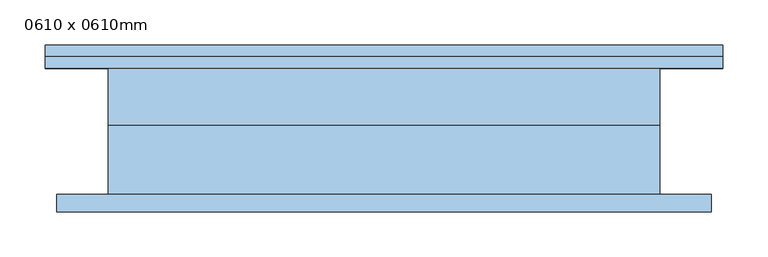
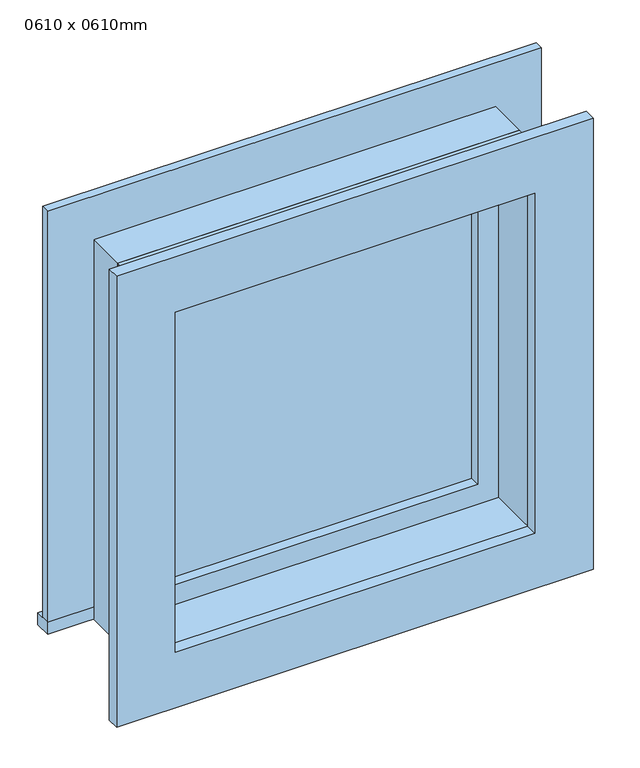
"""IFC4 building model written with IfcOpenShell, lengths in millimetres: window geometry, Travessa horizontal : 0610 x 0610mm."""

from ifc_helpers import new_model, si_unit, frame, origin, place, context, project, spatial, polyline, outline, extrude, source, transform, mapped, element, save


def window_0610_x_0610mm_59f802eb(model_context):
    return source(origin(), model_context, "Body", "SweptSolid", [
        extrude(outline(polyline([(-413.05, 95.7), (336.85, 95.7), (336.85, 70.0), (-413.05, 70.0), (-413.05, 95.7)])), frame((0.0, 0.0, 2159.0), z_axis=(0.0, 0.0, 1.0), x_axis=(1.0, 0.0, 0.0)), (0.0, 0.0, 1.0), 19.05),
        extrude(outline(polyline([(2749.95, -324.05), (2749.95, 247.85), (2178.05, 247.85), (2178.05, 336.85), (2838.95, 336.85), (2838.95, -413.05), (2178.05, -413.05), (2178.05, -324.05), (2749.95, -324.05)])), frame((0.0, 70.0, 0.0), z_axis=(0.0, 1.0, 0.0), x_axis=(0.0, 0.0, 1.0)), (0.0, 0.0, 1.0), 13.0),
        extrude(outline(polyline([(2826.25, 324.15), (2826.25, -400.35), (2101.75, -400.35), (2101.75, 324.15), (2826.25, 324.15)]), holes=[polyline([(2737.25, 235.15), (2190.75, 235.15), (2190.75, -311.35), (2737.25, -311.35), (2737.25, 235.15)])]), frame((0.0, -89.0, 0.0), z_axis=(0.0, 1.0, 0.0), x_axis=(0.0, 0.0, 1.0)), (0.0, 0.0, 1.0), 19.0),
        extrude(outline(polyline([(203.4, 22.425), (-279.6, 22.425), (-279.6, 35.125), (203.4, 35.125), (203.4, 22.425)])), frame((0.0, 0.0, 2222.5), z_axis=(0.0, 0.0, 1.0), x_axis=(1.0, 0.0, 0.0)), (0.0, 0.0, 1.0), 483.0),
        extrude(outline(polyline([(2749.95, -324.05), (2178.05, -324.05), (2178.05, 247.85), (2749.95, 247.85), (2749.95, -324.05)]), holes=[polyline([(2705.5, -279.6), (2705.5, 203.4), (2222.5, 203.4), (2222.5, -279.6), (2705.5, -279.6)])]), frame((0.0, 6.55, 0.0), z_axis=(0.0, 1.0, 0.0), x_axis=(0.0, 0.0, 1.0)), (0.0, 0.0, 1.0), 44.45),
        extrude(outline(polyline([(2769.0, -343.1), (2159.0, -343.1), (2159.0, 266.9), (2769.0, 266.9), (2769.0, -343.1)]), holes=[polyline([(2737.25, -311.35), (2737.25, 235.15), (2190.75, 235.15), (2190.75, -311.35), (2737.25, -311.35)])]), frame((0.0, -70.0, 0.0), z_axis=(0.0, 1.0, 0.0), x_axis=(0.0, 0.0, 1.0)), (0.0, 0.0, 1.0), 76.55),
        extrude(outline(polyline([(2769.0, 266.9), (2769.0, -343.1), (2159.0, -343.1), (2159.0, 266.9), (2769.0, 266.9)]), holes=[polyline([(2749.95, 247.85), (2178.05, 247.85), (2178.05, -324.05), (2749.95, -324.05), (2749.95, 247.85)])]), frame((0.0, 6.55, 0.0), z_axis=(0.0, 1.0, 0.0), x_axis=(0.0, 0.0, 1.0)), (0.0, 0.0, 1.0), 63.45),
    ])


if __name__ == "__main__":
    model = new_model("IFC4")
    model_context = context("Model", 3, world=origin())
    ifc_project = project(units=[si_unit("LENGTHUNIT", "METRE", prefix="MILLI")], contexts=[model_context])
    site = spatial("IfcSite", under=ifc_project)
    building = spatial("IfcBuilding", under=site)
    placement = place(None, origin())
    window_0610_x_0610mm_shape = window_0610_x_0610mm_59f802eb(model_context)
    element("IfcWindow", 1, ObjectType="Travessa horizontal : 0610 x 0610mm", at=placement, inside=building, context=model_context, shape_type="MappedRepresentation", body=[
        mapped(window_0610_x_0610mm_shape, transform((0.0, 0.0, 0.0), x_axis=(1.0, 0.0, 0.0), y_axis=(0.0, 1.0, 0.0), z_axis=(0.0, 0.0, 1.0))),
    ])
    save(model, "model.ifc")

# Revit data of these elements
# Type "Travessa horizontal : 0610 x 0610mm"
#   Type Mark = "EF31"
#   Construction Type Id = "GSP4R"
#   Analytic Construction = "Vidraça única Pilkington 1/8 pol"
#   Visual Light Transmittance = 0.9
#   Solar Heat Gain Coefficient = 0.78
#   Heat Transfer Coefficient (U) = 3.6886 W/(m²·K)
#   Height = 0.610 m
#   Altura-padrão do peitoril = 2.159 m
#   Projeção da apara - Ext. = 0.013 m
#   Projeção da apara - Int. = 0.019 m
#   Largura da apara - Exterior = 0.089 m
#   Largura da apara - Interior = 0.089 m
#   Width = 0.610 m
#   Janela aplicada = 0.019 m
#   Define Thermal Properties by = 1
#   Material do painel de vidro = Vidro
#   Material do caixilho = Caixilho
#   Material da apara externa = Recortar
#   Material da apara interna = Recortar
#   Wall Closure = (empty or 0)
# Element 1 (IfcWindow, "Travessa horizontal : 0610 x 0610mm")
#   Materials on its faces: "Recortar", "Caixilho", "Vidro"
# Materials
#   "Vidro": class "Vidro", colour RGB 0 128 192, transparency 0.9, Description = "Vidro de sílica", Cost = 0
#   "Caixilho": class "Madeira", colour RGB 224 178 126, transparency 0
#   "Recortar": class "Madeira", colour RGB 224 178 126, transparency 0
